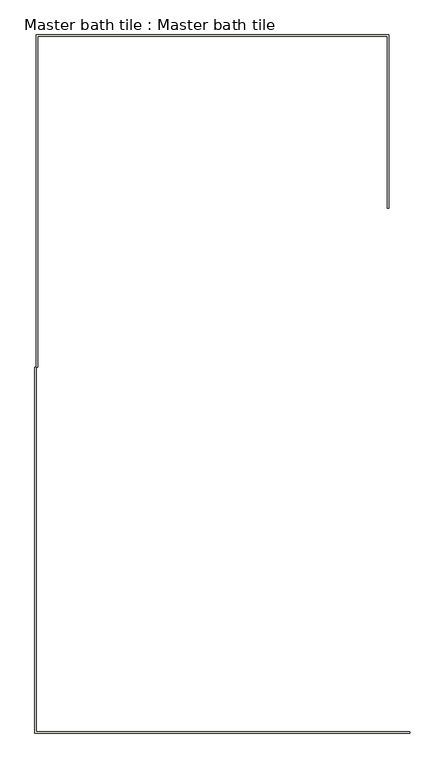
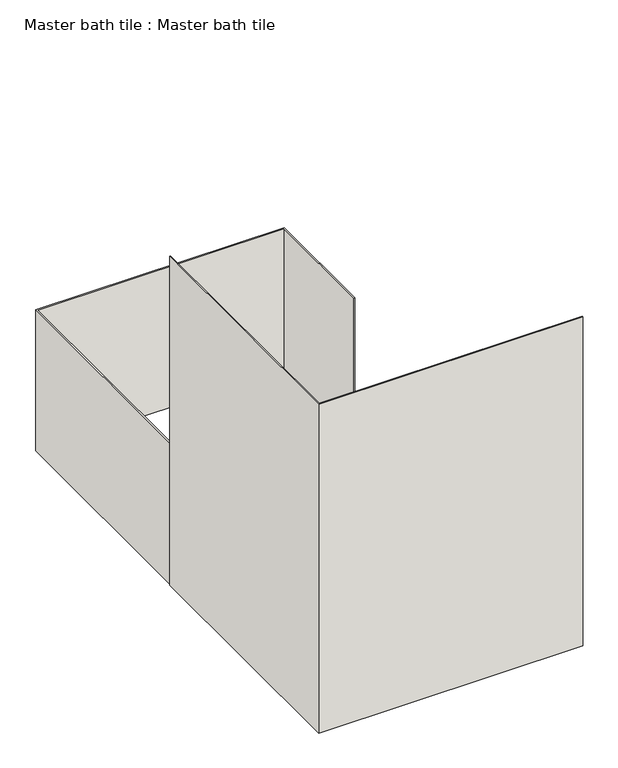
"""IFC4 building model written with IfcOpenShell, lengths in millimetres: wall geometry, Master bath tile : Master bath tile."""

import ifcopenshell
import ifcopenshell.guid

model = None  # the IFC model being written
_history = None  # IfcOwnerHistory: only IFC2X3 demands one
_inside = {}  # id of a spatial element -> (the spatial element, [elements in it])
_under = {}  # id of a project, library or spatial element -> (it, [spatial elements below it])
_declared = {}  # id of a project -> (the project, [libraries it declares])
_typed = {}  # id of a type object -> (the type object, [elements of that type])
_made_of = {}  # id of a material, layer set ... -> (it, [elements and type objects made of it])


def new_model(schema):
    """Start an empty IFC model of exactly this schema.

    Asked for "IFC4X3", IfcOpenShell would pick the latest addendum, in which some entities
    have other attributes; the version numbers below select the first issue.
    IFC2X3 requires an IfcOwnerHistory on every rooted entity: one is made here for all.
    """
    global model, _history
    if schema == "IFC4X3":
        model = ifcopenshell.file(schema_version=(4, 3, 0, 0))
    else:
        model = ifcopenshell.file(schema=schema)
    _inside.clear()
    _under.clear()
    _declared.clear()
    _typed.clear()
    _made_of.clear()
    _history = None
    if model.schema == "IFC2X3":
        org = make("IfcOrganization", Name="unknown")
        user = make(
            "IfcPersonAndOrganization",
            ThePerson=make("IfcPerson", FamilyName="unknown"),
            TheOrganization=org,
        )
        app = make(
            "IfcApplication",
            ApplicationDeveloper=org,
            Version="unknown",
            ApplicationFullName="unknown",
            ApplicationIdentifier="unknown",
        )
        _history = make(
            "IfcOwnerHistory",
            OwningUser=user,
            OwningApplication=app,
            ChangeAction="ADDED",
            CreationDate=0,
        )
    return model


def make(cls, **values):
    """One entity of the class cls with the attributes given. An attribute that is None is left unset."""
    return model.create_entity(
        cls, **{name: value for name, value in values.items() if value is not None}
    )


def rooted(cls, **values):
    """An entity with a GlobalId (a new one), such as an element, a storey or a relation."""
    return make(cls, GlobalId=ifcopenshell.guid.new(), OwnerHistory=_history, **values)


def si_unit(unit_type, name, prefix=None):
    """IfcSIUnit, for example si_unit("LENGTHUNIT", "METRE", prefix="MILLI")."""
    return make("IfcSIUnit", UnitType=unit_type, Prefix=prefix, Name=name)


def assignment(units):
    """IfcUnitAssignment: the units of a project."""
    return None if units is None else make("IfcUnitAssignment", Units=units)


def point(xyz):
    """IfcCartesianPoint."""
    return None if xyz is None else make("IfcCartesianPoint", Coordinates=xyz)


def direction(xyz):
    """IfcDirection."""
    return None if xyz is None else make("IfcDirection", DirectionRatios=xyz)


def frame(location, z_axis=None, x_axis=None):
    """IfcAxis2Placement3D, a coordinate frame: its origin and axes. An axis left out is left unset."""
    return make(
        "IfcAxis2Placement3D",
        Location=point(location),
        Axis=direction(z_axis),
        RefDirection=direction(x_axis),
    )


def origin():
    """The frame at (0, 0, 0) with its axes left unset."""
    return frame((0.0, 0.0, 0.0))


def origin_with_axes():
    """The frame at (0, 0, 0) with the z axis (0, 0, 1) and the x axis (1, 0, 0) written out."""
    return frame((0.0, 0.0, 0.0), z_axis=(0.0, 0.0, 1.0), x_axis=(1.0, 0.0, 0.0))


def place(relative_to, where):
    """IfcLocalPlacement: puts the frame where relative to a parent placement (None: the world)."""
    return make(
        "IfcLocalPlacement", PlacementRelTo=relative_to, RelativePlacement=where
    )


def context(
    kind, dimensions, precision=None, world=None, true_north=None, identifier=None
):
    """IfcGeometricRepresentationContext, for example the 3D "Model" context."""
    return make(
        "IfcGeometricRepresentationContext",
        ContextIdentifier=identifier,
        ContextType=kind,
        CoordinateSpaceDimension=dimensions,
        Precision=precision,
        WorldCoordinateSystem=world,
        TrueNorth=true_north,
    )


def project(units=None, contexts=None):
    """IfcProject with its units and contexts."""
    return rooted(
        "IfcProject",
        Name="project",
        RepresentationContexts=contexts,
        UnitsInContext=assignment(units),
    )


def spatial(cls, under=None, at=None, **own):
    """A site, building, storey or space (cls), placed at a placement, below another one or the project."""
    s = rooted(cls, ObjectPlacement=at, **own)
    if under is not None:
        _under.setdefault(under.id(), (under, []))[1].append(s)
    return s


def polyline(points):
    """IfcPolyline through the points."""
    return make("IfcPolyline", Points=[point(p) for p in points])


def outline(outer, holes=None, kind="AREA"):
    """IfcArbitraryClosedProfileDef: a profile drawn as a closed curve; with holes, ...WithVoids."""
    if holes is None:
        return make("IfcArbitraryClosedProfileDef", ProfileType=kind, OuterCurve=outer)
    return make(
        "IfcArbitraryProfileDefWithVoids",
        ProfileType=kind,
        OuterCurve=outer,
        InnerCurves=holes,
    )


def extrude(swept, where, along, depth):
    """IfcExtrudedAreaSolid: the profile swept, set in the frame where, extruded along a direction by depth."""
    return make(
        "IfcExtrudedAreaSolid",
        SweptArea=swept,
        Position=where,
        ExtrudedDirection=direction(along),
        Depth=depth,
    )


def shape(context_of_items, identifier, shape_type, items):
    """IfcShapeRepresentation: the items that make up one representation, for example the "Body"."""
    return make(
        "IfcShapeRepresentation",
        ContextOfItems=context_of_items,
        RepresentationIdentifier=identifier,
        RepresentationType=shape_type,
        Items=items,
    )


def source(mapping_origin, context_of_items, identifier, shape_type, items):
    """IfcRepresentationMap: a shape defined once, which mapped items show again and again."""
    return make(
        "IfcRepresentationMap",
        MappingOrigin=mapping_origin,
        MappedRepresentation=shape(context_of_items, identifier, shape_type, items),
    )


def transform(
    local_origin,
    x_axis=None,
    y_axis=None,
    z_axis=None,
    scale=None,
    scale2=None,
    scale3=None,
    uniform=True,
):
    """IfcCartesianTransformationOperator3D, or its non-uniform kind. x_axis, y_axis, z_axis: its Axis1, 2, 3."""
    if uniform:
        return make(
            "IfcCartesianTransformationOperator3D",
            Axis1=direction(x_axis),
            Axis2=direction(y_axis),
            LocalOrigin=point(local_origin),
            Scale=scale,
            Axis3=direction(z_axis),
        )
    return make(
        "IfcCartesianTransformationOperator3DnonUniform",
        Axis1=direction(x_axis),
        Axis2=direction(y_axis),
        LocalOrigin=point(local_origin),
        Scale=scale,
        Axis3=direction(z_axis),
        Scale2=scale2,
        Scale3=scale3,
    )


def mapped(mapping_source, mapping_target):
    """IfcMappedItem: shows the shape of a source again, moved by a transform."""
    return make(
        "IfcMappedItem", MappingSource=mapping_source, MappingTarget=mapping_target
    )


def made_of(thing, what):
    """Note that an element or type object is made of a material, layer set ...; save() writes the relation."""
    if what is not None:
        _made_of.setdefault(what.id(), (what, []))[1].append(thing)
    return thing


def element(
    cls,
    number,
    at=None,
    inside=None,
    cuts=None,
    type_object=None,
    material=None,
    context=None,
    identifier="Body",
    shape_type=None,
    held_by="IfcProductDefinitionShape",
    body=None,
    shapes=None,
    **own,
):
    """One element of the class cls, such as IfcWall. Its Tag is "e" and its number.

    at: its placement. inside: the storey or other place that contains it. cuts: it is an
    opening in that element (IfcRelVoidsElement). A single representation is given by context,
    identifier, shape_type and body (its items); several are given by shapes. held_by: the class
    of the entity that holds the representations. save() writes the other relations.
    """
    e = rooted(cls, Tag="e%d" % number, ObjectPlacement=at, **own)
    if body is not None:
        shapes = [shape(context, identifier, shape_type, body)]
    if shapes is not None:
        e.Representation = make(held_by, Representations=shapes)
    if inside is not None:
        _inside.setdefault(inside.id(), (inside, []))[1].append(e)
    if cuts is not None:
        rooted(
            "IfcRelVoidsElement", RelatingBuildingElement=cuts, RelatedOpeningElement=e
        )
    if type_object is not None:
        _typed.setdefault(type_object.id(), (type_object, []))[1].append(e)
    return made_of(e, material)


def aggregate(whole, parts):
    """IfcRelAggregates: a whole, such as a stair, and the parts it consists of."""
    return rooted("IfcRelAggregates", RelatingObject=whole, RelatedObjects=parts)


def save(model, path):
    """Write the relations noted so far, then the file.

    IfcRelAggregates (storeys below a building ...), IfcRelContainedInSpatialStructure (elements
    in a storey), IfcRelDefinesByType, IfcRelAssociatesMaterial and IfcRelDeclares: one each for
    every whole, place, type object, material and project.
    """
    for whole, parts in _under.values():
        aggregate(whole, parts)
    for where, things in _inside.values():
        rooted(
            "IfcRelContainedInSpatialStructure",
            RelatedElements=things,
            RelatingStructure=where,
        )
    for kind, things in _typed.values():
        rooted("IfcRelDefinesByType", RelatedObjects=things, RelatingType=kind)
    for what, things in _made_of.values():
        rooted("IfcRelAssociatesMaterial", RelatedObjects=things, RelatingMaterial=what)
    for by, libraries in _declared.values():
        rooted("IfcRelDeclares", RelatingContext=by, RelatedDefinitions=libraries)
    model.write(path)


def master_bath_tile_master_bath_tile_4ed34d6c(model_context):
    return source(origin(), model_context, "Body", "SweptSolid", [
        extrude(outline(polyline([(-10225.0875, 15727.3625), (-8701.0875, 15727.3625), (-8701.0875, 14978.0625), (-8707.4375, 14978.0625), (-8707.4375, 15721.0125), (-10218.7375, 15721.0125), (-10218.7375, 14292.2625), (-10225.0875, 14292.2625), (-10225.0875, 15727.3625)])), origin_with_axes(), (0.0, 0.0, 1.0), 914.4),
        extrude(outline(polyline([(-10231.4375, 12712.7), (-10231.4375, 14293.2375), (-10225.0875, 14293.2375), (-10225.0875, 12719.05), (-8610.6, 12719.05), (-8610.6, 12712.7), (-10231.4375, 12712.7)])), origin_with_axes(), (0.0, 0.0, 1.0), 2133.6),
    ])


if __name__ == "__main__":
    model = new_model("IFC4")
    model_context = context("Model", 3, world=origin())
    ifc_project = project(units=[si_unit("LENGTHUNIT", "METRE", prefix="MILLI")], contexts=[model_context])
    site = spatial("IfcSite", under=ifc_project)
    building = spatial("IfcBuilding", under=site)
    placement = place(None, origin())
    master_bath_tile_master_bath_tile_shape = master_bath_tile_master_bath_tile_4ed34d6c(model_context)
    element("IfcWall", 1, ObjectType="Master bath tile : Master bath tile", at=placement, inside=building, context=model_context, shape_type="MappedRepresentation", body=[
        mapped(master_bath_tile_master_bath_tile_shape, transform((0.0, 0.0, 0.0), x_axis=(1.0, 0.0, 0.0), y_axis=(0.0, 1.0, 0.0), z_axis=(0.0, 0.0, 1.0))),
    ])
    save(model, "model.ifc")

# Revit data of these elements
# Type "Master bath tile : Master bath tile"
#   COBie.Type = no
# Element 1 (IfcWall, "Master bath tile : Master bath tile")
#   Materials on its faces: "Tile, grey Green"
# Materials
#   "Tile, grey Green": class "Generic", colour RGB 70 104 106, transparency 0, Description = "Porcelain tile, 4\", white", Cost = 0
